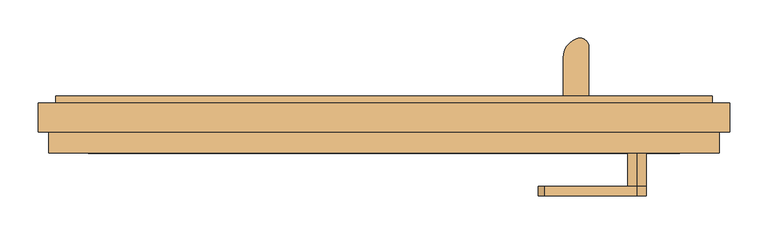
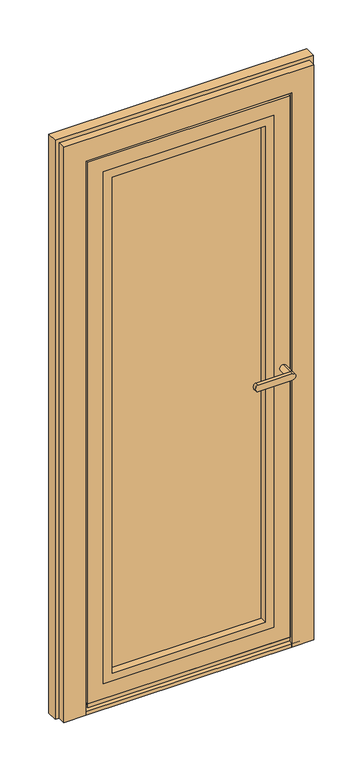
"""IFC4 building model written with IfcOpenShell, lengths in millimetres: door geometry, Schueco_FWS_ADS-75-BL-SimplySmart_out_Family-01 : FWS SI insert unit."""

from ifc_helpers import new_model, si_unit, point, frame, frame_2d, origin, place, context, project, spatial, polyline, circle_curve, ellipse_curve, trimmed, segment, composite_curve, outline, extrude, faceted_brep, source, transform, mapped, element, save
from ifc_brep_helpers import plane_surface, cylinder_surface, extruded_surface, advanced_brep


def door_9c0b083d(model_context):
    return source(origin(), model_context, "Body", "SolidModel", [
        extrude(outline(composite_curve([segment(polyline([(235.3327032, 9.0), (235.3327032, 59.1621505)]), True, "CONTINUOUS"), segment(trimmed(circle_curve(frame_2d((262.5111209, 59.1621505)), 27.1784177), [point((235.3327032, 59.1621505))], [point((252.9740253, 84.6123017))], False, "CARTESIAN"), True, "CONTINUOUS"), segment(trimmed(circle_curve(frame_2d((257.0515262, 73.7313144)), 11.6198924), [point((252.9740253, 84.6123017))], [point((268.6714186, 73.7313144))], False, "CARTESIAN"), True, "CONTINUOUS"), segment(polyline([(268.6714186, 73.7313144), (268.6714186, 9.0), (235.3327032, 9.0)]), True, "CONTINUOUS")], self_intersect=False)), frame((0.0, 0.0, 2030.9340013), z_axis=(0.0, 0.0, 1.0), x_axis=(1.0, 0.0, 0.0)), (0.0, 0.0, 1.0), 4.0),
        extrude(outline(polyline([(235.3327032, 13.0), (268.6714186, 13.0), (268.6714186, 9.0), (235.3327032, 9.0), (235.3327032, 13.0)])), frame((0.0, 0.0, 2000.9340013), z_axis=(0.0, 0.0, 1.0), x_axis=(1.0, 0.0, 0.0)), (0.0, 0.0, 1.0), 30.0),
        extrude(outline(polyline([(235.3327032, 13.0), (268.6714186, 13.0), (268.6714186, 9.0), (235.3327032, 9.0), (235.3327032, 13.0)])), frame((0.0, 0.0, 56.9340013), z_axis=(0.0, 0.0, 1.0), x_axis=(1.0, 0.0, 0.0)), (0.0, 0.0, 1.0), 30.0),
        extrude(outline(composite_curve([segment(polyline([(235.3327032, 9.0), (235.3327032, 59.1621505)]), True, "CONTINUOUS"), segment(trimmed(circle_curve(frame_2d((262.5111209, 59.1621505)), 27.1784177), [point((235.3327032, 59.1621505))], [point((252.9740253, 84.6123017))], False, "CARTESIAN"), True, "CONTINUOUS"), segment(trimmed(circle_curve(frame_2d((257.0515262, 73.7313144)), 11.6198924), [point((252.9740253, 84.6123017))], [point((268.6714186, 73.7313144))], False, "CARTESIAN"), True, "CONTINUOUS"), segment(polyline([(268.6714186, 73.7313144), (268.6714186, 9.0), (235.3327032, 9.0)]), True, "CONTINUOUS")], self_intersect=False)), frame((0.0, 0.0, 52.9340013), z_axis=(0.0, 0.0, 1.0), x_axis=(1.0, 0.0, 0.0)), (0.0, 0.0, 1.0), 4.0),
        advanced_brep(
        [(264.7171028, 57.5980002, 2030.9340013), (239.2829507, 72.2824248, 2030.9340013), (264.7171028, 57.5980002, 56.9340013), (239.2829507, 72.2824248, 56.9340013)],
        [
            (0, 1, ellipse_curve(frame((252.0000268, 64.9402125, 2030.9340013), z_axis=(0.0, 0.0, 1.0), x_axis=(0.5000002582658956, 0.866025254674503, 0.0)), 21.5840887, 14.6844171)),
            (1, 0, ellipse_curve(frame((252.0000268, 64.9402125, 2030.9340013), z_axis=(0.0, 0.0, 1.0), x_axis=(0.5000002582658956, 0.866025254674503, 0.0)), 21.5840887, 14.6844171)),
            (2, 3, ellipse_curve(frame((252.0000268, 64.9402125, 56.9340013), z_axis=(0.0, 0.0, -1.0), x_axis=(-0.866025254674503, 0.5000002582658956, 0.0)), 14.6844171, 21.5840887)),
            (3, 2, ellipse_curve(frame((252.0000268, 64.9402125, 56.9340013), z_axis=(0.0, 0.0, -1.0), x_axis=(-0.866025254674503, 0.5000002582658956, 0.0)), 14.6844171, 21.5840887)),
            (0, 2),
            (3, 1),
        ],
        [
            plane_surface(frame((239.2829507, 72.2824248, 2030.9340013), z_axis=(0.0, 0.0, 1.0), x_axis=(0.5000002582658956, 0.866025254674503, 0.0))),
            plane_surface(frame((239.2829507, 72.2824248, 56.9340013), z_axis=(0.0, 0.0, -1.0), x_axis=(-0.5000002582658956, -0.866025254674503, 0.0))),
            extruded_surface(trimmed(ellipse_curve(frame((252.0000268, 64.9402125, 56.9340013), z_axis=(0.0, 0.0, -1.0), x_axis=(-0.866025254674503, 0.5000002582658956, 0.0)), 14.6844171, 21.5840887), [point((239.2829507, 72.2824248, 56.9340013))], [point((264.7171028, 57.5980002, 56.9340013))], True, "CARTESIAN"), (0.0, 0.0, -1974.0), 1974.0),
            extruded_surface(trimmed(ellipse_curve(frame((252.0000268, 64.9402125, 56.9340013), z_axis=(0.0, 0.0, -1.0), x_axis=(-0.866025254674503, 0.5000002582658956, 0.0)), 14.6844171, 21.5840887), [point((264.7171028, 57.5980002, 56.9340013))], [point((239.2829507, 72.2824248, 56.9340013))], True, "CARTESIAN"), (0.0, 0.0, -1974.0), 1974.0),
        ],
        [
            (0, [[1, 2]]),
            (1, [[3, 4]]),
            (2, [[5, -4, 6, -1]]),
            (3, [[-6, -3, -5, -2]]),
        ],
    ),
        advanced_brep(
        [(332.0000268, -121.9999695, 1038.0113692), (332.0000268, -121.9999695, 1061.9886308), (210.3382342, -121.9999695, 1061.9886308), (210.3382342, -121.9999695, 1038.0113692), (332.0000268, -109.4998825, 1061.9886308), (332.0000268, -109.4998825, 1038.0113692), (210.3382342, -109.4998825, 1038.0113692), (210.3382342, -109.4998825, 1061.9886308), (332.0000268, -66.0, 1038.0113692), (332.0000268, -66.0, 1061.9886308)],
        [
            (0, 1, circle_curve(frame((332.0000268, -121.9999695, 1050.0), z_axis=(0.0, -1.0, 0.0), x_axis=(0.0, 0.0, 1.0)), 11.9886308)),
            (1, 2),
            (2, 3, ellipse_curve(frame((210.3382342, -121.9999695, 1050.0), z_axis=(0.0, -1.0, 0.0), x_axis=(0.0, 0.0, -1.0)), 11.9886308, 7.9050795)),
            (3, 0),
            (4, 5, circle_curve(frame((332.0000268, -109.4998825, 1050.0), z_axis=(0.0, -1.0, 0.0), x_axis=(0.0, 0.0, 1.0)), 11.9886308)),
            (5, 6),
            (6, 7, ellipse_curve(frame((210.3382342, -109.4998825, 1050.0), z_axis=(0.0, 1.0, 0.0), x_axis=(0.0, 0.0, -1.0)), 11.9886308, 7.9050795)),
            (7, 4),
            (3, 6),
            (5, 0),
            (2, 7),
            (1, 4),
            (5, 4, circle_curve(frame((332.0000268, -109.4998825, 1050.0), z_axis=(0.0, -1.0, 0.0), x_axis=(0.0, 0.0, 1.0)), 11.9886308)),
            (8, 9, circle_curve(frame((332.0000268, -66.0, 1050.0), z_axis=(0.0, 1.0, 0.0), x_axis=(0.0, 0.0, 1.0)), 11.9886308)),
            (9, 8, circle_curve(frame((332.0000268, -66.0, 1050.0), z_axis=(0.0, 1.0, 0.0), x_axis=(0.0, 0.0, 1.0)), 11.9886308)),
            (8, 5),
            (4, 9),
        ],
        [
            plane_surface(frame((210.3382342, -121.9999695, 1038.0113692), z_axis=(0.0, -1.0, 0.0), x_axis=(-1.0, 0.0, 0.0))),
            plane_surface(frame((210.3382342, -109.4998825, 1038.0113692), z_axis=(0.0, 1.0, 0.0), x_axis=(1.0, 0.0, 0.0))),
            plane_surface(frame((332.0000268, -121.9999695, 1038.0113692), z_axis=(0.0, 0.0, -1.0), x_axis=(0.0, 1.0, 0.0))),
            extruded_surface(trimmed(ellipse_curve(frame((210.3382342, -109.4998825, 1050.0), z_axis=(0.0, 1.0, 0.0), x_axis=(0.0, 0.0, -1.0)), 11.9886308, 7.9050795), [point((210.3382342, -109.4998825, 1038.0113692))], [point((210.3382342, -109.4998825, 1061.9886308))], True, "CARTESIAN"), (0.0, 12.500086999999994, 0.0), 12.500086999999994),
            plane_surface(frame((210.3382342, -121.9999695, 1061.9886308), z_axis=(0.0, 0.0, 1.0), x_axis=(0.0, 1.0, 0.0))),
            cylinder_surface(frame((332.0000268, -109.4998825, 1050.0), z_axis=(0.0, -1.0, 0.0), x_axis=(0.0, 0.0, 1.0)), 11.9886308),
            plane_surface(frame((332.0000268, -66.0, 1061.9886308), z_axis=(0.0, 1.0, 0.0), x_axis=(-1.0, 0.0, 0.0))),
            cylinder_surface(frame((332.0000268, -66.0, 1050.0), z_axis=(0.0, -1.0, 0.0), x_axis=(0.0, 0.0, 1.0)), 11.9886308),
        ],
        [
            (0, [[1, 2, 3, 4]]),
            (1, [[5, 6, 7, 8]]),
            (2, [[9, -6, 10, -4]]),
            (3, [[11, -7, -9, -3]]),
            (4, [[12, -8, -11, -2]]),
            (5, [[-10, 13, -12, -1]]),
            (6, [[14, 15]]),
            (7, [[16, -5, 17, -14]]),
            (7, [[-17, -13, -16, -15]]),
        ],
    ),
        extrude(outline(polyline([(95.0, 300.0000268), (2000.0, 300.0000268), (2000.0, -299.9999732), (95.0, -299.9999732), (95.0, 300.0000268)]), holes=[polyline([(125.0, -269.9999732), (1970.0, -269.9999732), (1970.0, 270.0000268), (125.0, 270.0000268), (125.0, -269.9999732)])]), frame((0.0, -66.0, 0.0), z_axis=(0.0, 1.0, 0.0), x_axis=(0.0, 0.0, 1.0)), (0.0, 0.0, 1.0), 26.0000097),
        faceted_brep([(-354.9999732, -66.0, 2055.0), (-354.9999732, -57.4997243, 2055.0), (-354.9999732, -57.4997243, 40.0), (-354.9999732, -66.0, 40.0), (355.0000268, -57.4997243, 40.0), (355.0000268, -66.0, 40.0), (365.0000268, -57.4997243, 30.0), (365.0000268, -57.4997243, 2065.0), (-364.9999732, -57.4997243, 2065.0), (-364.9999732, -57.4997243, 30.0), (355.0000268, -57.4997243, 2055.0), (355.0000268, -66.0, 2055.0), (-299.9999732, -66.0, 95.0), (-299.9999732, -66.0, 2000.0), (300.0000268, -66.0, 2000.0), (300.0000268, -66.0, 95.0), (-299.9999732, -1.9999903, 2000.0), (-299.9999732, -1.9999903, 95.0), (300.0000268, -1.9999903, 95.0), (300.0000268, -1.9999903, 2000.0), (-267.9999732, -1.9999903, 127.0), (-267.9999732, -1.9999903, 1968.0), (268.0000268, -1.9999903, 1968.0), (268.0000268, -1.9999903, 127.0), (-267.9999732, 9.0, 1968.0), (-267.9999732, 9.0, 127.0), (268.0000268, 9.0, 127.0), (268.0000268, 9.0, 1968.0), (-386.9981317, 9.0, 8.0018415), (-386.9981317, 9.0, 2086.9981585), (386.9981853, 9.0, 2086.9981585), (386.9981853, 9.0, 8.0018415), (-386.9981317, 0.5000426, 2086.9981585), (-386.9981317, 0.5000426, 8.0018415), (386.9981853, 0.5000426, 8.0018415), (386.9981853, 0.5000426, 2086.9981585), (-364.9999732, 0.5000426, 30.0), (-364.9999732, 0.5000426, 2065.0), (365.0000268, 0.5000426, 2065.0), (365.0000268, 0.5000426, 30.0)], [[[0, 1, 2, 3]], [[3, 2, 4, 5]], [[6, 7, 8, 9], [2, 1, 10, 4]], [[5, 4, 10, 11]], [[5, 11, 0, 3], [12, 13, 14, 15]], [[16, 13, 12, 17]], [[17, 12, 15, 18]], [[18, 15, 14, 19]], [[18, 19, 16, 17], [20, 21, 22, 23]], [[24, 21, 20, 25]], [[25, 20, 23, 26]], [[26, 23, 22, 27]], [[28, 29, 30, 31], [26, 27, 24, 25]], [[32, 29, 28, 33]], [[33, 28, 31, 34]], [[34, 31, 30, 35]], [[34, 35, 32, 33], [36, 37, 38, 39]], [[8, 37, 36, 9]], [[9, 36, 39, 6]], [[6, 39, 38, 7]], [[11, 10, 1, 0]], [[19, 14, 13, 16]], [[27, 22, 21, 24]], [[35, 30, 29, 32]], [[7, 38, 37, 8]]]),
        extrude(outline(polyline([(300.0000268, -39.9999903), (-299.9999732, -39.9999903), (-299.9999732, -1.9999903), (300.0000268, -1.9999903), (300.0000268, -39.9999903)])), frame((0.0, 0.0, 95.0), z_axis=(0.0, 0.0, 1.0), x_axis=(1.0, 0.0, 0.0)), (0.0, 0.0, 1.0), 1905.0),
        extrude(outline(polyline([(-354.9999732, -66.0), (-354.9999732, -57.4997243), (355.0000268, -57.4997243), (355.0000268, -66.0), (-354.9999732, -66.0)])), frame((0.0, 0.0, 26.0), z_axis=(0.0, 0.0, 1.0), x_axis=(1.0, 0.0, 0.0)), (0.0, 0.0, 1.0), 14.0),
        faceted_brep([(430.999943, 8.9997177, 2130.999943), (430.999943, 0.0, 2130.999943), (430.999943, 0.0, 0.0), (430.999943, 8.9997177, 0.0), (-454.0, 0.0, 0.0), (-454.0, 0.0, 2154.0), (454.0, 0.0, 2154.0), (454.0, 0.0, 0.0), (-430.999943, 0.0, 2130.999943), (-430.999943, 0.0, 0.0), (454.0, -38.0, 0.0), (440.0, -38.0, 0.0), (440.0, -66.0002823, 0.0), (361.9999732, -66.0002823, 0.0), (361.9999732, -57.5000065, 0.0), (388.4999732, -57.5000065, 0.0), (388.4999732, 0.4997603, 0.0), (393.9999732, 0.4997603, 0.0), (393.9999732, 8.9997177, 0.0), (-393.9999732, 8.9997177, 0.0), (-430.999943, 8.9997177, 0.0), (-430.999943, 8.9997177, 2130.999943), (393.9999732, 8.9997177, 2093.9999732), (-393.9999732, 8.9997177, 2093.9999732), (361.9999732, -66.0002823, 2061.9999732), (361.9999732, -57.5000065, 2061.9999732), (-361.9999732, -57.5000065, 0.0), (-388.4999732, -57.5000065, 0.0), (-388.4999732, -57.5000065, 2088.4999732), (388.4999732, -57.5000065, 2088.4999732), (-361.9999732, -57.5000065, 2061.9999732), (-440.0, -66.0002823, 0.0), (-361.9999732, -66.0002823, 0.0), (-361.9999732, -66.0002823, 2061.9999732), (440.0, -66.0002823, 2140.0), (-440.0, -66.0002823, 2140.0), (440.0, -38.0, 2140.0), (-454.0, -38.0, 0.0), (-440.0, -38.0, 0.0), (-440.0, -38.0, 2140.0), (454.0, -38.0, 2154.0), (-454.0, -38.0, 2154.0), (-393.9999732, 0.4997603, 0.0), (-388.4999732, 0.4997603, 0.0), (393.9999732, 0.4997603, 2093.9999732), (-393.9999732, 0.4997603, 2093.9999732), (388.4999732, 0.4997603, 2088.4999732), (-388.4999732, 0.4997603, 2088.4999732)], [[[0, 1, 2, 3]], [[4, 5, 6, 7, 2, 1, 8, 9]], [[3, 2, 7, 10, 11, 12, 13, 14, 15, 16, 17, 18]], [[19, 20, 21, 0, 3, 18, 22, 23]], [[24, 25, 14, 13]], [[26, 27, 28, 29, 15, 14, 25, 30]], [[31, 32, 33, 24, 13, 12, 34, 35]], [[34, 12, 11, 36]], [[37, 38, 39, 36, 11, 10, 40, 41]], [[4, 9, 20, 19, 42, 43, 27, 26, 32, 31, 38, 37]], [[20, 9, 8, 21]], [[18, 17, 44, 22]], [[42, 19, 23, 45]], [[32, 26, 30, 33]], [[31, 35, 39, 38]], [[4, 37, 41, 5]], [[6, 40, 10, 7]], [[43, 42, 45, 44, 17, 16, 46, 47]], [[16, 15, 29, 46]], [[27, 43, 47, 28]], [[21, 8, 1, 0]], [[33, 30, 25, 24]], [[35, 34, 36, 39]], [[23, 22, 44, 45]], [[5, 41, 40, 6]], [[47, 46, 29, 28]]]),
        extrude(outline(polyline([(0.5000426, 16.5), (0.5000426, 0.0), (-66.0002823, 0.0), (-66.0002823, 13.2855157), (-46.5000038, 20.0), (-44.0000038, 20.0), (-44.0000038, 16.5), (0.5000426, 16.5)])), frame((-388.4999732, 0.0, 0.0), z_axis=(1.0, 0.0, 0.0), x_axis=(0.0, 1.0, 0.0)), (0.0, 0.0, 1.0), 776.9999465),
    ])


if __name__ == "__main__":
    model = new_model("IFC4")
    model_context = context("Model", 3, world=origin())
    ifc_project = project(units=[si_unit("LENGTHUNIT", "METRE", prefix="MILLI")], contexts=[model_context])
    site = spatial("IfcSite", under=ifc_project)
    building = spatial("IfcBuilding", under=site)
    placement = place(None, origin())
    door_shape = door_9c0b083d(model_context)
    element("IfcDoor", 1, ObjectType="Schueco_FWS_ADS-75-BL-SimplySmart_out_Family-01 : FWS SI insert unit", at=placement, inside=building, context=model_context, shape_type="MappedRepresentation", body=[
        mapped(door_shape, transform((0.0, 0.0, 0.0), x_axis=(1.0, 0.0, 0.0), y_axis=(0.0, 1.0, 0.0), z_axis=(0.0, 0.0, 1.0))),
    ])
    save(model, "model.ifc")

# Revit data of these elements
# Type "Schueco_FWS_ADS-75-BL-SimplySmart_out_Family-01 : FWS SI insert unit"
#   Type Mark = "31"
#   __NOTE___ = "Data describes the optimum values of the entire system. The properites of a selected design option have to be determined on an individual basis!"
#   Wind load resistance = "Class C3"
#   Watertightness = "Class E750"
#   Thermal insulation = "Uf = 1.6 W/(m²K)"
#   Sound insulation = "..."
#   Schueco thermal insulation standard = "Highly thermally insulated"
#   Opening type = "Outward-opening, Flush-fitted"
#   Model = "Schueco ADS 75 BL SimplySmart"
#   Mechanical loading = "..."
#   Maximum leaf width in mm = "1400"
#   Maximum leaf weight in kg = "200"
#   Maximum leaf height in mm = "3000"
#   Material = "Aluminium"
#   Construction Type = "Door, single-leaf, outward-opening"
#   Manufacturer = "Schueco International KG"
#   Long term functionality = "..."
#   Glazing data = "Triple glazing 38mm"
#   Façade insert unit = "yes"
#   Family creation date = "08.2017"
#   Description = "Schueco Aluminium Door System (ADS)"
#   Burglar resistance = "Class RC 2"
#   Areas of use = "Public buildings, Residential buildings, Side entrance"
#   Analytic Construction = "<None>"
#   Air permeability = "Class 4"
#   Width [instance default] = 1053.69 mm
#   Leaf opening angle [instance default] = 0.00°
#   IOf_T = 38 mm
#   Height [instance default] = 1928.68 mm
#   Glazing area [instance default] = 1.10139 m²
#   Distance from bottom to handles [instance default] = 1050 mm
#   Clear opening width [instance default] = 869.69 mm
#   Standard threshold = yes
#   Low level threshold = no
#   Handles = yes
#   FWS SI insert unit = yes
#   FWS HI insert unit = no
#   Glass = none
#   Frame = Alu
#   Fittings = none
# Element 1 (IfcDoor, "Schueco_FWS_ADS-75-BL-SimplySmart_out_Family-01 : FWS SI insert unit")
#   Width = 908 mm
#   Height = 2154 mm
#   Glazing area = 0.986776 m²
#   Clear opening width = 724 mm
#   Materials on its faces: "Alu", "Glass"
# Materials
#   "Alu": class "Glas", colour RGB 140 140 140, transparency 0
#   "Glass": class "Glass", colour RGB 128 128 255, transparency 0.75, Description = "Soda Lime Glass", Cost = 0
